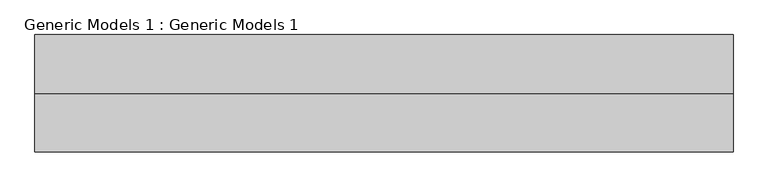
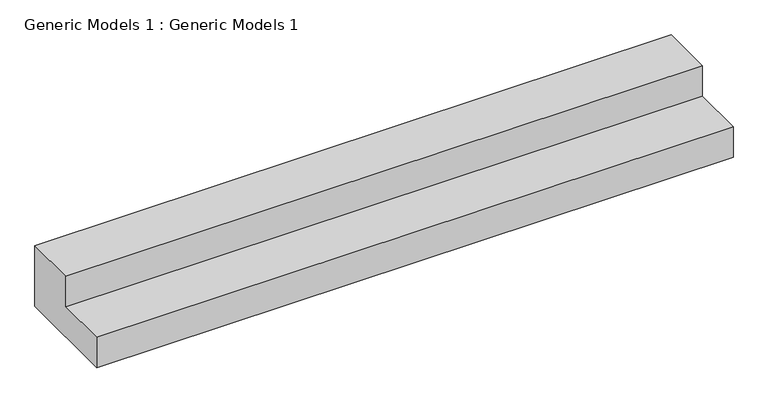
"""IFC4 building model written with IfcOpenShell, lengths in millimetres: proxy geometry, Generic Models 1 : Generic Models 1."""

from ifc_helpers import new_model, si_unit, frame, origin, place, context, project, spatial, polyline, outline, extrude, source, transform, mapped, element, save


def generic_models_1_generic_models_1_43cdfc79(model_context):
    return source(origin(), model_context, "Body", "SweptSolid", [
        extrude(outline(polyline([(788.2914588, 300.0), (1038.2914588, 300.0), (1038.2914588, 0.0), (538.2914588, 0.0), (538.2914588, 150.0), (788.2914588, 150.0), (788.2914588, 300.0)])), frame((-11849.2253352, 0.0, 0.0), z_axis=(1.0, 0.0, 0.0), x_axis=(0.0, 1.0, 0.0)), (0.0, 0.0, 1.0), 2970.0),
    ])


if __name__ == "__main__":
    model = new_model("IFC4")
    model_context = context("Model", 3, world=origin())
    ifc_project = project(units=[si_unit("LENGTHUNIT", "METRE", prefix="MILLI")], contexts=[model_context])
    site = spatial("IfcSite", under=ifc_project)
    building = spatial("IfcBuilding", under=site)
    placement = place(None, origin())
    generic_models_1_generic_models_1_shape = generic_models_1_generic_models_1_43cdfc79(model_context)
    element("IfcBuildingElementProxy", 1, Name="Generic Models 1 : Generic Models 1", ObjectType="Generic Models 1 : Generic Models 1", at=placement, inside=building, context=model_context, shape_type="MappedRepresentation", body=[
        mapped(generic_models_1_generic_models_1_shape, transform((0.0, 0.0, 0.0), x_axis=(1.0, 0.0, 0.0), y_axis=(0.0, 1.0, 0.0), z_axis=(0.0, 0.0, 1.0))),
    ])
    save(model, "model.ifc")
